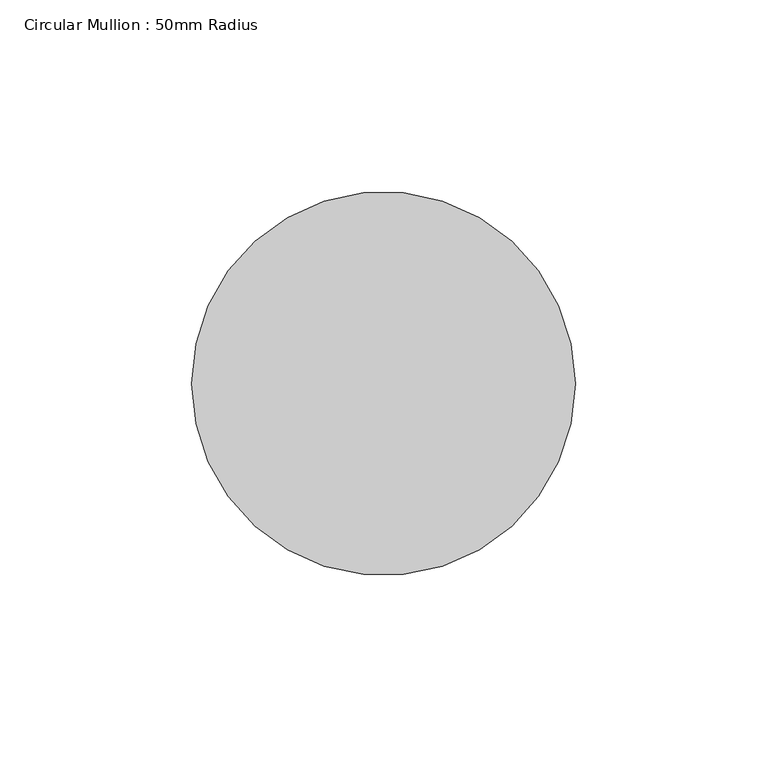
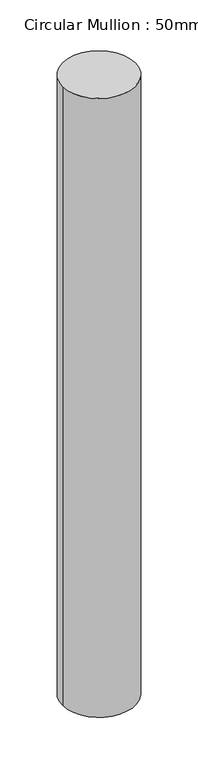
"""IFC4 building model written with IfcOpenShell, lengths in millimetres: member geometry, Circular Mullion : 50mm Radius."""

from ifc_helpers import new_model, si_unit, point, frame, origin, origin_2d, place, context, project, spatial, circle_curve, trimmed, segment, composite_curve, outline, extrude, source, transform, mapped, element, save


def circular_mullion_50mm_radius_bf03cfd7(model_context):
    return source(origin(), model_context, "Body", "SweptSolid", [
        extrude(outline(composite_curve([segment(trimmed(circle_curve(origin_2d(), 50.0), [point((50.0, 0.0))], [point((-50.0, 0.0))], False, "CARTESIAN"), True, "CONTINUOUS"), segment(trimmed(circle_curve(origin_2d(), 50.0), [point((-50.0, 0.0))], [point((50.0, 0.0))], False, "CARTESIAN"), True, "CONTINUOUS")], self_intersect=False)), frame((0.0, 0.0, -903.4781335), z_axis=(0.0, 0.0, 1.0), x_axis=(1.0, 0.0, 0.0)), (0.0, 0.0, 1.0), 903.4781335),
    ])


if __name__ == "__main__":
    model = new_model("IFC4")
    model_context = context("Model", 3, world=origin())
    ifc_project = project(units=[si_unit("LENGTHUNIT", "METRE", prefix="MILLI")], contexts=[model_context])
    site = spatial("IfcSite", under=ifc_project)
    building = spatial("IfcBuilding", under=site)
    placement = place(None, origin())
    circular_mullion_50mm_radius_shape = circular_mullion_50mm_radius_bf03cfd7(model_context)
    element("IfcMember", 1, ObjectType="Circular Mullion : 50mm Radius", at=placement, inside=building, context=model_context, shape_type="MappedRepresentation", body=[
        mapped(circular_mullion_50mm_radius_shape, transform((0.0, 0.0, 0.0), x_axis=(1.0, 0.0, 0.0), y_axis=(0.0, 1.0, 0.0), z_axis=(0.0, 0.0, 1.0))),
    ])
    save(model, "model.ifc")

# Revit data of these elements
# Type "Circular Mullion : 50mm Radius"
#   built-in parameter 1007350 = 0.164042 (stored number, unit not read)
# Element 1 (IfcMember, "Circular Mullion : 50mm Radius")
#   Materials on its faces: "Aluminium"
# Materials
#   "Aluminium": class "Metal", colour RGB 247 247 247, transparency 0, Description = "Aluminium 6061", Cost = 0
